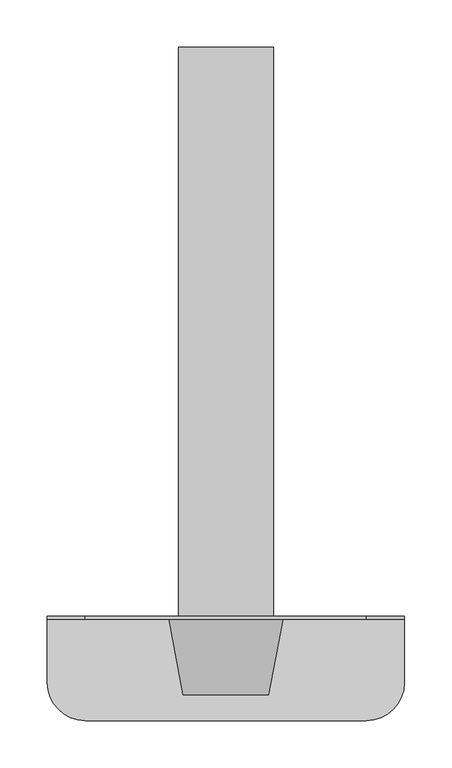
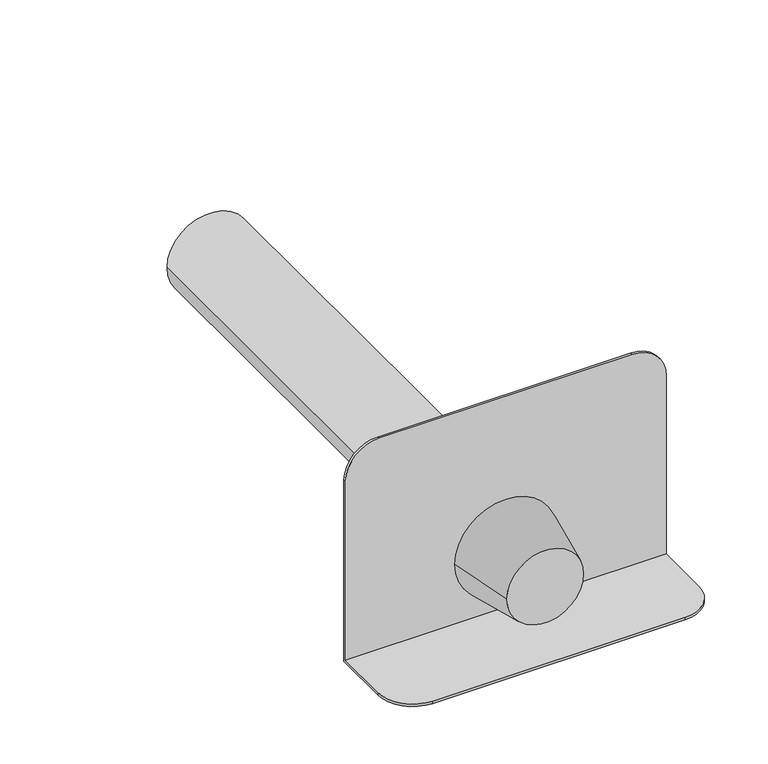
"""IFC4 building model written with IfcOpenShell, lengths in millimetres: proxy geometry, TN_Воронка парапетная ТехноНИКОЛЬ круглая_Тип 1 : Воронка парапетная ТехноНИКОЛЬ (круглого сечения) 110х600."""

from ifc_helpers import new_model, si_unit, frame, origin, place, context, project, spatial, polyline, circle_curve, source, transform, mapped, element, save
from ifc_brep_helpers import plane_surface, cylinder_surface, revolved_surface, advanced_brep


def specialty_equipment_d8b1a70e(model_context):
    return source(origin(), model_context, "Body", "AdvancedBrep", [
        advanced_brep(
        [(-45.0, -83.0, 77.0), (45.0, -83.0, 77.0), (-60.0, -3.0, 77.0), (60.0, -3.0, 77.0)],
        [
            (0, 1, circle_curve(frame((0.0, -83.0, 77.0), z_axis=(0.0, -1.0, 0.0), x_axis=(-1.0, 0.0, 0.0)), 45.0)),
            (1, 0, circle_curve(frame((0.0, -83.0, 77.0), z_axis=(0.0, -1.0, 0.0), x_axis=(1.0, 0.0, 0.0)), 45.0)),
            (2, 3, circle_curve(frame((0.0, -3.0, 77.0), z_axis=(0.0, 1.0, 0.0), x_axis=(1.0, 0.0, 0.0)), 60.0)),
            (3, 2, circle_curve(frame((0.0, -3.0, 77.0), z_axis=(0.0, 1.0, 0.0), x_axis=(-1.0, 0.0, 0.0)), 60.0)),
            (3, 1),
            (0, 2),
        ],
        [
            plane_surface(frame((0.0, -83.0, 77.0), z_axis=(0.0, -1.0, 0.0), x_axis=(0.0, 0.0, -1.0))),
            plane_surface(frame((0.0, -3.0, 77.0), z_axis=(0.0, 1.0, 0.0), x_axis=(0.0, 0.0, -1.0))),
            revolved_surface(polyline([(-45.0, -83.0, 77.0), (-60.0, -3.0, 77.0)]), (0.0, -323.0, 77.0), (0.0, 1.0, 0.0)),
            revolved_surface(polyline([(45.0, -83.0, 77.0), (60.0, -3.0, 77.0)]), (0.0, -323.0, 77.0), (0.0, 1.0, 0.0)),
        ],
        [
            (0, [[1, 2]]),
            (1, [[3, 4]]),
            (2, [[-4, 5, -1, 6]]),
            (3, [[-3, -6, -2, -5]]),
        ],
    ),
        advanced_brep(
        [(-188.5, -70.0, 3.0), (-148.5, -110.0, 3.0), (148.5, -110.0, 3.0), (188.5, -70.0, 3.0), (188.5, -3.0, 3.0), (-188.5, -3.0, 3.0), (-188.5, 0.0, 0.0), (188.5, 0.0, 0.0), (188.5, -70.0, 0.0), (148.5, -110.0, 0.0), (-148.5, -110.0, 0.0), (-188.5, -70.0, 0.0), (188.5, 0.0, 225.0), (188.5, -3.0, 225.0), (-188.5, 0.0, 225.0), (-148.5, 0.0, 265.0), (148.5, 0.0, 265.0), (-50.0, 0.0, 77.0), (50.0, 0.0, 77.0), (-188.5, -3.0, 225.0), (148.5, -3.0, 265.0), (-148.5, -3.0, 265.0), (-47.0, -3.0, 77.0), (47.0, -3.0, 77.0), (-47.0, 0.0, 77.0), (47.0, 0.0, 77.0), (-50.0, 600.0, 77.0), (50.0, 600.0, 77.0), (-47.0, 600.0, 77.0), (47.0, 600.0, 77.0)],
        [
            (0, 1, circle_curve(frame((-148.5, -70.0, 3.0), z_axis=(0.0, 0.0, 1.0), x_axis=(1.0, 0.0, 0.0)), 40.0)),
            (1, 2),
            (2, 3, circle_curve(frame((148.5, -70.0, 3.0), z_axis=(0.0, 0.0, 1.0), x_axis=(1.0, 0.0, 0.0)), 40.0)),
            (3, 4),
            (4, 5),
            (5, 0),
            (6, 7),
            (7, 8),
            (8, 9, circle_curve(frame((148.5, -70.0, 0.0), z_axis=(0.0, 0.0, -1.0), x_axis=(1.0, 0.0, 0.0)), 40.0)),
            (9, 10),
            (10, 11, circle_curve(frame((-148.5, -70.0, 0.0), z_axis=(0.0, 0.0, -1.0), x_axis=(1.0, 0.0, 0.0)), 40.0)),
            (11, 6),
            (0, 11),
            (10, 1),
            (9, 2),
            (8, 3),
            (7, 12),
            (12, 13),
            (13, 4),
            (6, 14),
            (14, 15, circle_curve(frame((-148.5, 0.0, 225.0), z_axis=(0.0, 1.0, 0.0), x_axis=(1.0, 0.0, 0.0)), 40.0)),
            (15, 16),
            (16, 12, circle_curve(frame((148.5, 0.0, 225.0), z_axis=(0.0, 1.0, 0.0), x_axis=(1.0, 0.0, 0.0)), 40.0)),
            (17, 18, circle_curve(frame((0.0, 0.0, 77.0), z_axis=(0.0, -1.0, 0.0), x_axis=(1.0, 0.0, 0.0)), 50.0)),
            (18, 17, circle_curve(frame((0.0, 0.0, 77.0), z_axis=(0.0, -1.0, 0.0), x_axis=(1.0, 0.0, 0.0)), 50.0)),
            (5, 19),
            (19, 14),
            (13, 20, circle_curve(frame((148.5, -3.0, 225.0), z_axis=(0.0, -1.0, 0.0), x_axis=(1.0, 0.0, 0.0)), 40.0)),
            (20, 21),
            (21, 19, circle_curve(frame((-148.5, -3.0, 225.0), z_axis=(0.0, -1.0, 0.0), x_axis=(1.0, 0.0, 0.0)), 40.0)),
            (22, 23, circle_curve(frame((0.0, -3.0, 77.0), z_axis=(0.0, 1.0, 0.0), x_axis=(1.0, 0.0, 0.0)), 47.0)),
            (23, 22, circle_curve(frame((0.0, -3.0, 77.0), z_axis=(0.0, 1.0, 0.0), x_axis=(1.0, 0.0, 0.0)), 47.0)),
            (16, 20),
            (15, 21),
            (22, 24),
            (24, 25, circle_curve(frame((0.0, 0.0, 77.0), z_axis=(0.0, 1.0, 0.0), x_axis=(1.0, 0.0, 0.0)), 47.0)),
            (25, 23),
            (25, 24, circle_curve(frame((0.0, 0.0, 77.0), z_axis=(0.0, 1.0, 0.0), x_axis=(1.0, 0.0, 0.0)), 47.0)),
            (26, 27, circle_curve(frame((0.0, 600.0, 77.0), z_axis=(0.0, 1.0, 0.0), x_axis=(1.0, 0.0, 0.0)), 50.0)),
            (27, 26, circle_curve(frame((0.0, 600.0, 77.0), z_axis=(0.0, 1.0, 0.0), x_axis=(1.0, 0.0, 0.0)), 50.0)),
            (28, 29, circle_curve(frame((0.0, 600.0, 77.0), z_axis=(0.0, -1.0, 0.0), x_axis=(1.0, 0.0, 0.0)), 47.0)),
            (29, 28, circle_curve(frame((0.0, 600.0, 77.0), z_axis=(0.0, -1.0, 0.0), x_axis=(1.0, 0.0, 0.0)), 47.0)),
            (27, 18),
            (17, 26),
            (29, 25),
            (24, 28),
        ],
        [
            plane_surface(frame((-108.5, -70.0, 3.0), z_axis=(0.0, 0.0, 1.0), x_axis=(0.0, 1.0, 0.0))),
            plane_surface(frame((-108.5, -70.0, 0.0), z_axis=(0.0, 0.0, -1.0), x_axis=(0.0, -1.0, 0.0))),
            cylinder_surface(frame((-148.5, -70.0, 0.0), z_axis=(0.0, 0.0, 1.0), x_axis=(1.0, 0.0, 0.0)), 40.0),
            plane_surface(frame((-148.5, -110.0, 3.0), z_axis=(0.0, -1.0, 0.0), x_axis=(0.0, 0.0, -1.0))),
            cylinder_surface(frame((148.5, -70.0, 0.0), z_axis=(0.0, 0.0, 1.0), x_axis=(1.0, 0.0, 0.0)), 40.0),
            plane_surface(frame((188.5, -70.0, 3.0), z_axis=(1.0, 0.0, 0.0), x_axis=(0.0, 0.0, -1.0))),
            plane_surface(frame((188.5, 0.0, 3.0), z_axis=(0.0, 1.0, 0.0), x_axis=(0.0, 0.0, -1.0))),
            plane_surface(frame((-188.5, 0.0, 3.0), z_axis=(-1.0, 0.0, 0.0), x_axis=(0.0, 0.0, -1.0))),
            plane_surface(frame((-188.5, -3.0, 0.0), z_axis=(0.0, -1.0, 0.0), x_axis=(1.0, 0.0, 0.0))),
            cylinder_surface(frame((148.5, 0.0, 225.0), z_axis=(0.0, -1.0, 0.0), x_axis=(1.0, 0.0, 0.0)), 40.0),
            plane_surface(frame((148.5, -3.0, 265.0), z_axis=(0.0, 0.0, 1.0), x_axis=(0.0, 1.0, 0.0))),
            cylinder_surface(frame((-148.5, 0.0, 225.0), z_axis=(0.0, -1.0, 0.0), x_axis=(1.0, 0.0, 0.0)), 40.0),
            revolved_surface(polyline([(47.0, 0.0, 77.0), (47.0, -3.0, 77.0)]), (0.0, 0.0, 77.0), (0.0, 1.0, 0.0)),
            plane_surface(frame((50.0, 600.0, 77.0), z_axis=(0.0, 1.0, 0.0), x_axis=(0.0, 0.0, -1.0))),
            cylinder_surface(frame((0.0, 600.0, 77.0), z_axis=(0.0, -1.0, 0.0), x_axis=(1.0, 0.0, 0.0)), 50.0),
            revolved_surface(polyline([(47.0, 600.0, 77.0), (47.0, 0.0, 77.0)]), (0.0, 0.0, 77.0), (0.0, 1.0, 0.0)),
        ],
        [
            (0, [[1, 2, 3, 4, 5, 6]]),
            (1, [[7, 8, 9, 10, 11, 12]]),
            (2, [[-1, 13, -11, 14]]),
            (3, [[-2, -14, -10, 15]]),
            (4, [[-3, -15, -9, 16]]),
            (5, [[-16, -8, 17, 18, 19, -4]]),
            (6, [[-7, 20, 21, 22, 23, -17], [24, 25]]),
            (7, [[-13, -6, 26, 27, -20, -12]]),
            (8, [[28, 29, 30, -26, -5, -19], [31, 32]]),
            (9, [[-28, -18, -23, 33]]),
            (10, [[-29, -33, -22, 34]]),
            (11, [[-30, -34, -21, -27]]),
            (12, [[-31, 35, 36, 37]]),
            (12, [[-32, -37, 38, -35]]),
            (13, [[39, 40], [41, 42]]),
            (14, [[-40, 43, -24, 44]]),
            (14, [[-39, -44, -25, -43]]),
            (15, [[-42, 45, -36, 46]]),
            (15, [[-41, -46, -38, -45]]),
        ],
    ),
    ])


if __name__ == "__main__":
    model = new_model("IFC4")
    model_context = context("Model", 3, world=origin())
    ifc_project = project(units=[si_unit("LENGTHUNIT", "METRE", prefix="MILLI")], contexts=[model_context])
    site = spatial("IfcSite", under=ifc_project)
    building = spatial("IfcBuilding", under=site)
    placement = place(None, origin())
    specialty_equipment_shape = specialty_equipment_d8b1a70e(model_context)
    element("IfcBuildingElementProxy", 1, Name="TN_Воронка парапетная ТехноНИКОЛЬ круглая_Тип 1 : Воронка парапетная ТехноНИКОЛЬ (круглого сечения) 110х600", ObjectType="TN_Воронка парапетная ТехноНИКОЛЬ круглая_Тип 1 : Воронка парапетная ТехноНИКОЛЬ (круглого сечения) 110х600", at=placement, inside=building, context=model_context, shape_type="MappedRepresentation", body=[
        mapped(specialty_equipment_shape, transform((0.0, 0.0, 0.0), x_axis=(1.0, 0.0, 0.0), y_axis=(0.0, 1.0, 0.0), z_axis=(0.0, 0.0, 1.0))),
    ])
    save(model, "model.ifc")

# Revit data of these elements
# Type "TN_Воронка парапетная ТехноНИКОЛЬ круглая_Тип 1 : Воронка парапетная ТехноНИКОЛЬ (круглого сечения) 110х600"
#   ADSK_Группирование = "Комплектующие и воронки"
#   Description = "Кровельная воронка для отвода воды через кровельные или балконные парапеты"
#   Manufacturer = "ТехноНИКОЛЬ"
#   URL = "https://nav.tn.ru/catalog/krovlya/vodostochnaya-sistema/parapetnaya-voronka-tekhnonikol/"
#   ADSK_Примечание = ""
#   ADSK_Обозначение = "ТехноНИКОЛЬ"
#   ADSK_Наименование = "Воронка парапетная ТехноНИКОЛЬ (круглого сечения) 110х600мм"
#   ADSK_Марка = ""
#   ADSK_Код изделия = "52496"
#   ADSK_Завод-изготовитель = "ТехноНИКОЛЬ"
#   ADSK_Единица измерения = "шт."
#   ADSK_Группирование = "Комплектующие и воронки"
#   ADSK_URL страницы изделия = "https://nav.tn.ru/catalog/krovlya/vodostochnaya-sistema/parapetnaya-voronka-tekhnonikol/"
#   ADSK_URL документации изделия = ""
#   Ширина фланца = 377 mm
#   Размер фланца по вертикали = 265 mm
#   Длина расчетная [instance default] = 600 mm
#   Длина отвода [instance default] = 600 mm
#   Размер фланца по горизонтали = 110 mm
#   ADSK_Масса = 0.5
#   ADSK_Количество = 1
#   Тип воронки = 2
#   Видимость_Переход [instance default] = no
#   Видимость_Листоуловитель [instance default] = no
#   Материал = TN_ПВХ_Черный
#   Default Elevation = 0
# Element 1 (IfcBuildingElementProxy, "TN_Воронка парапетная ТехноНИКОЛЬ круглая_Тип 1 : Воронка парапетная ТехноНИКОЛЬ (круглого сечения) 110х600")
#   Видимость_Переход = yes
#   Видимость_Листоуловитель = yes
#   Materials on its faces: "TN_ПВХ_Черный"
# Materials
#   "TN_ПВХ_Черный": class "Типовые", colour RGB 48 48 48, transparency 0, Cost = 0
